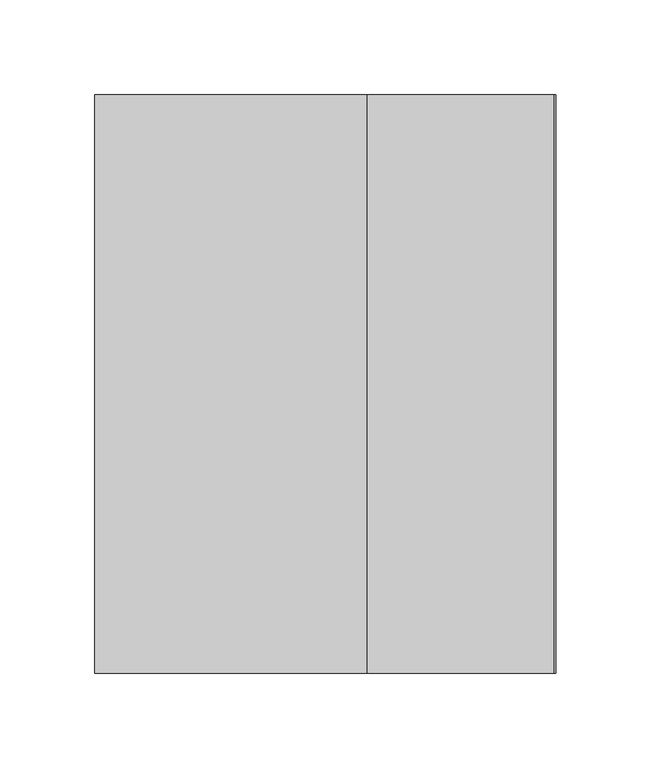
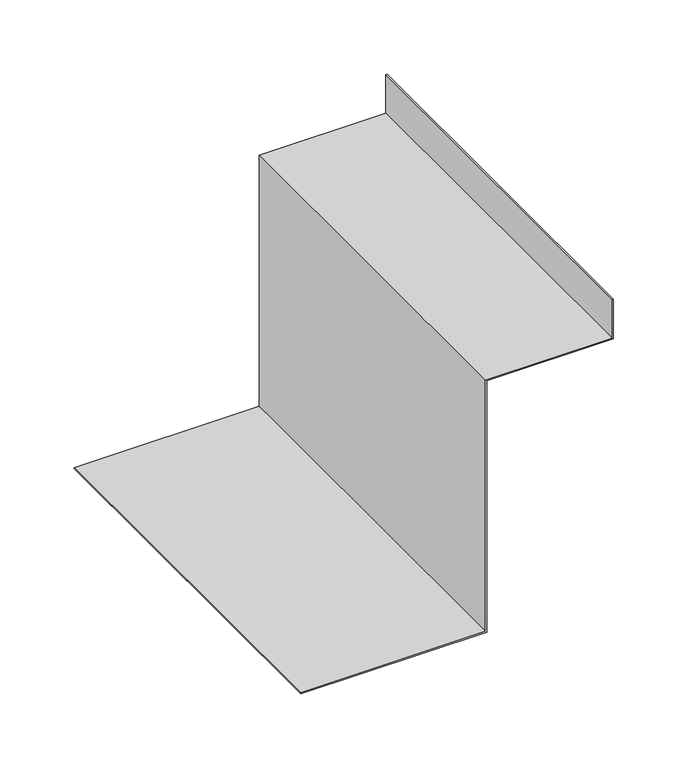
"""IFC4 building model written with IfcOpenShell, lengths in millimetres: proxy geometry, Generic Models 335:Generic Models 335:155398 : Generic Models 335:Generic Models 335:155398."""

from ifc_helpers import new_model, si_unit, frame, origin, place, context, project, spatial, polyline, outline, extrude, source, transform, mapped, element, save


def generic_models_5299e789(model_context):
    return source(origin(), model_context, "Body", "SweptSolid", [
        extrude(outline(polyline([(3097.0430926, 8532.7671126), (3065.2930926, 8532.7671126), (3065.2930926, 8434.1571753), (2858.9025119, 8434.1571753), (2858.9025119, 8290.5286548), (2857.9890616, 8290.5286548), (2857.9890616, 8435.0825739), (3064.5124204, 8435.0825739), (3064.5124204, 8533.6082629), (3097.0430926, 8533.6082629), (3097.0430926, 8532.7671126)])), frame((0.0, -3919.5173293, 0.0), z_axis=(0.0, 1.0, 0.0), x_axis=(0.0, 0.0, 1.0)), (0.0, 0.0, 1.0), 304.8),
    ])


if __name__ == "__main__":
    model = new_model("IFC4")
    model_context = context("Model", 3, world=origin())
    ifc_project = project(units=[si_unit("LENGTHUNIT", "METRE", prefix="MILLI")], contexts=[model_context])
    site = spatial("IfcSite", under=ifc_project)
    building = spatial("IfcBuilding", under=site)
    placement = place(None, origin())
    generic_models_shape = generic_models_5299e789(model_context)
    element("IfcBuildingElementProxy", 1, Name="Generic Models 335:Generic Models 335:155398 : Generic Models 335:Generic Models 335:155398", ObjectType="Generic Models 335:Generic Models 335:155398 : Generic Models 335:Generic Models 335:155398", at=placement, inside=building, context=model_context, shape_type="MappedRepresentation", body=[
        mapped(generic_models_shape, transform((0.0, 0.0, 0.0), x_axis=(1.0, 0.0, 0.0), y_axis=(0.0, 1.0, 0.0), z_axis=(0.0, 0.0, 1.0))),
    ])
    save(model, "model.ifc")

# Revit data of these elements
# Type "Generic Models 335:Generic Models 335:155398 : Generic Models 335:Generic Models 335:155398"
#   NameOverride = "Generic Models 335:Generic Models 335:155398"
#   ObjectTypeOverride = "Generic Models 335:Generic Models 335"
#   Reference = "Generic Models 335"
#   Category = "Generic Models"
#   Tag = "155398"
# Element 1 (IfcBuildingElementProxy, "Generic Models 335:Generic Models 335:155398 : Generic Models 335:Generic Models 335:155398")
#   Materials on its faces: "_(2) LAYERS NO. 30 ASTM D226 ASPHALT SATURATED ORGANIC FELT 997"
# Materials
#   "_(2) LAYERS NO. 30 ASTM D226 ASPHALT SATURATED ORGANIC FELT 997": class "Unassigned", colour RGB 67 154 161, transparency 0
